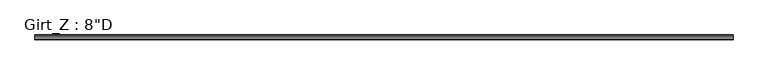
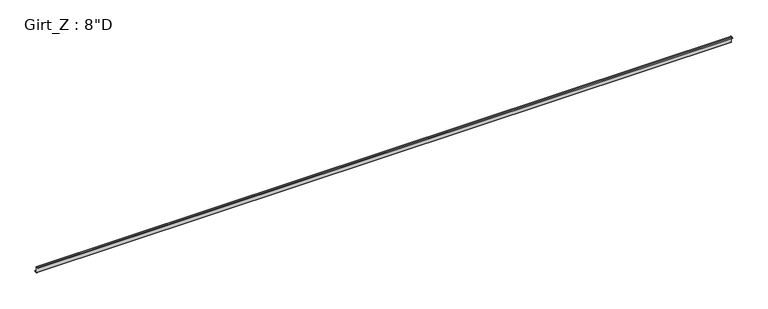
"""IFC4 building model written with IfcOpenShell, lengths in millimetres: beam geometry."""

from ifc_helpers import new_model, si_unit, point, frame, frame_2d, origin, place, context, project, spatial, polyline, circle_curve, trimmed, segment, composite_curve, outline, extrude, source, transform, mapped, element, save


def beam_739fbb00(model_context):
    return source(origin(), model_context, "Body", "SweptSolid", [
        extrude(outline(composite_curve([segment(polyline([(-63.5, 101.6), (-3.3734375, 101.6)]), True, "CONTINUOUS"), segment(trimmed(circle_curve(frame_2d((-3.3734375, 96.8375)), 4.7625), [point((-3.3734375, 101.6))], [point((1.3890625, 96.8375))], False, "CARTESIAN"), True, "CONTINUOUS"), segment(polyline([(1.3890625, 96.8375), (1.3890625, -96.8389339)]), True, "CONTINUOUS"), segment(trimmed(circle_curve(frame_2d((3.3748024, -96.8389339)), 1.9857399), [point((1.3890625, -96.8389339))], [point((3.2694106, -98.821875))], True, "CARTESIAN"), True, "CONTINUOUS"), segment(polyline([(3.2694106, -98.821875), (62.204539, -98.821875), (73.6169367, -85.221109), (75.745104, -87.0068534), (63.5, -101.6), (3.3734375, -101.6)]), True, "CONTINUOUS"), segment(trimmed(circle_curve(frame_2d((3.3734375, -96.8375)), 4.7625), [point((3.3734375, -101.6))], [point((-1.3890625, -96.8375))], False, "CARTESIAN"), True, "CONTINUOUS"), segment(polyline([(-1.3890625, -96.8375), (-1.3890625, 96.8381931)]), True, "CONTINUOUS"), segment(trimmed(circle_curve(frame_2d((-3.3741066, 96.8381931)), 1.9850441), [point((-1.3890625, 96.8381931))], [point((-3.3005807, 98.821875))], True, "CARTESIAN"), True, "CONTINUOUS"), segment(polyline([(-3.3005807, 98.821875), (-62.204539, 98.821875), (-73.6169367, 85.221109), (-75.745104, 87.0068534), (-63.5, 101.6)]), True, "CONTINUOUS")], self_intersect=False)), frame((-10972.8, 0.0, 0.0), z_axis=(1.0, 0.0, 0.0), x_axis=(0.0, 1.0, 0.0)), (0.0, 0.0, 1.0), 21831.7960937),
    ])


if __name__ == "__main__":
    model = new_model("IFC4")
    model_context = context("Model", 3, world=origin())
    ifc_project = project(units=[si_unit("LENGTHUNIT", "METRE", prefix="MILLI")], contexts=[model_context])
    site = spatial("IfcSite", under=ifc_project)
    building = spatial("IfcBuilding", under=site)
    placement = place(None, origin())
    beam_shape = beam_739fbb00(model_context)
    element("IfcBeam", 1, ObjectType="Girt_Z : 8\"D", at=placement, inside=building, context=model_context, shape_type="MappedRepresentation", body=[
        mapped(beam_shape, transform((0.0, 0.0, 0.0), x_axis=(1.0, 0.0, 0.0), y_axis=(0.0, 1.0, 0.0), z_axis=(0.0, 0.0, 1.0))),
    ])
    save(model, "model.ifc")

# Revit data of these elements
# Type "Girt_Z : 8\"D"
#   Web_Thickness = 0' - 0 7/64"
#   Length [instance default] = 10' - 0"
#   Leg_1 = 0' - 2 1/2"
#   Height = 0' - 8"
#   Structural Material [instance default] = none
# Element 1 (IfcBeam, "Girt_Z : 8\"D")
#   Structural Material = Steel
#   Materials on its faces: "Steel"
# Materials
#   "Steel": class "Metal", colour RGB 118 118 114, transparency 0, Description = "Steel, mill finish", Cost = 0
